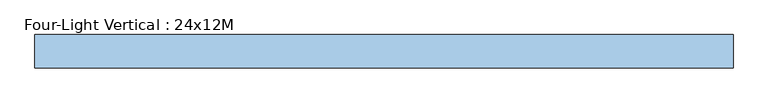
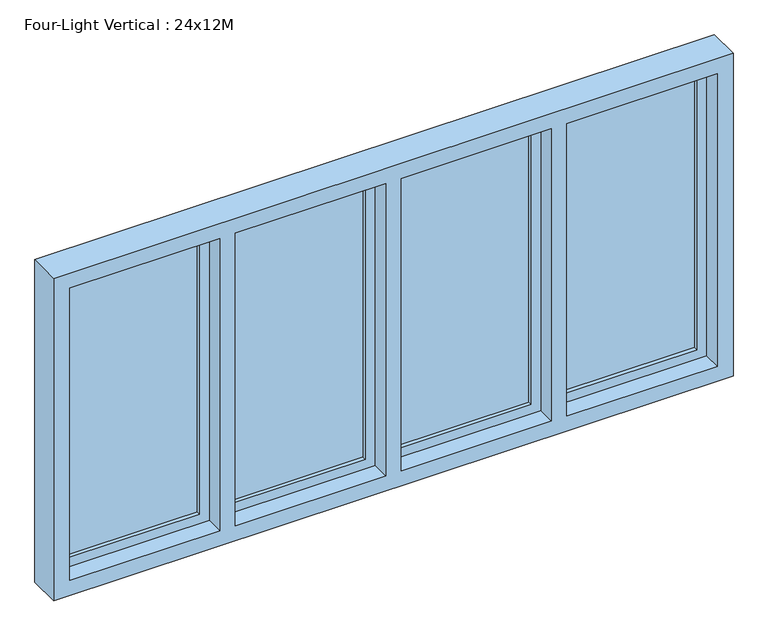
"""IFC4 building model written with IfcOpenShell, lengths in millimetres: window geometry, Four-Light Vertical : 24x12M."""

from ifc_helpers import new_model, si_unit, frame, origin, place, context, project, spatial, polyline, outline, extrude, faceted_brep, source, transform, mapped, element, save


def four_light_vertical_24x12m_47221696(model_context):
    return source(origin(), model_context, "Body", "SolidModel", [
        extrude(outline(polyline([(1970.0, -1224.0), (842.0, -1224.0), (842.0, -660.75), (1970.0, -660.75), (1970.0, -1224.0)]), holes=[polyline([(1920.0, -710.75), (892.0, -710.75), (892.0, -1174.0), (1920.0, -1174.0), (1920.0, -710.75)])]), frame((0.0, 134.0, 0.0), z_axis=(0.0, 1.0, 0.0), x_axis=(0.0, 0.0, 1.0)), (0.0, 0.0, 1.0), 50.0),
        extrude(outline(polyline([(1970.0, -635.75), (842.0, -635.75), (842.0, -72.5), (1970.0, -72.5), (1970.0, -635.75)]), holes=[polyline([(1920.0, -122.5), (892.0, -122.5), (892.0, -585.75), (1920.0, -585.75), (1920.0, -122.5)])]), frame((0.0, 134.0, 0.0), z_axis=(0.0, 1.0, 0.0), x_axis=(0.0, 0.0, 1.0)), (0.0, 0.0, 1.0), 50.0),
        extrude(outline(polyline([(1970.0, -47.5), (842.0, -47.5), (842.0, 515.75), (1970.0, 515.75), (1970.0, -47.5)]), holes=[polyline([(1920.0, 465.75), (892.0, 465.75), (892.0, 2.5), (1920.0, 2.5), (1920.0, 465.75)])]), frame((0.0, 134.0, 0.0), z_axis=(0.0, 1.0, 0.0), x_axis=(0.0, 0.0, 1.0)), (0.0, 0.0, 1.0), 50.0),
        extrude(outline(polyline([(1970.0, 540.75), (842.0, 540.75), (842.0, 1104.0), (1970.0, 1104.0), (1970.0, 540.75)]), holes=[polyline([(1920.0, 1054.0), (892.0, 1054.0), (892.0, 590.75), (1920.0, 590.75), (1920.0, 1054.0)])]), frame((0.0, 134.0, 0.0), z_axis=(0.0, 1.0, 0.0), x_axis=(0.0, 0.0, 1.0)), (0.0, 0.0, 1.0), 50.0),
        faceted_brep([(-1266.0, 184.0, 800.0), (1146.0, 184.0, 800.0), (1146.0, 69.0, 800.0), (-1266.0, 69.0, 800.0), (1146.0, 184.0, 2012.0), (1146.0, 69.0, 2012.0), (-1266.0, 184.0, 2012.0), (1104.0, 184.0, 842.0), (1104.0, 184.0, 1970.0), (540.75, 184.0, 1970.0), (540.75, 184.0, 842.0), (-1224.0, 184.0, 1970.0), (-1224.0, 184.0, 842.0), (-660.75, 184.0, 842.0), (-660.75, 184.0, 1970.0), (515.75, 184.0, 842.0), (515.75, 184.0, 1970.0), (-47.5, 184.0, 1970.0), (-47.5, 184.0, 842.0), (-72.5, 184.0, 1970.0), (-635.75, 184.0, 1970.0), (-635.75, 184.0, 842.0), (-72.5, 184.0, 842.0), (-1266.0, 69.0, 2012.0), (1089.0, 69.0, 1955.0), (1089.0, 69.0, 857.0), (555.75, 69.0, 857.0), (555.75, 69.0, 1955.0), (500.75, 69.0, 1955.0), (500.75, 69.0, 857.0), (-32.5, 69.0, 857.0), (-32.5, 69.0, 1955.0), (-87.5, 69.0, 857.0), (-620.75, 69.0, 857.0), (-620.75, 69.0, 1955.0), (-87.5, 69.0, 1955.0), (-1209.0, 69.0, 857.0), (-1209.0, 69.0, 1955.0), (-675.75, 69.0, 1955.0), (-675.75, 69.0, 857.0), (1089.0, 134.0, 857.0), (555.75, 134.0, 857.0), (-1209.0, 134.0, 857.0), (-675.75, 134.0, 857.0), (500.75, 134.0, 857.0), (-32.5, 134.0, 857.0), (-87.5, 134.0, 857.0), (-620.75, 134.0, 857.0), (1089.0, 134.0, 1955.0), (1104.0, 134.0, 1970.0), (1104.0, 134.0, 842.0), (540.75, 134.0, 842.0), (540.75, 134.0, 1970.0), (555.75, 134.0, 1955.0), (-1224.0, 134.0, 842.0), (-1224.0, 134.0, 1970.0), (-660.75, 134.0, 1970.0), (-660.75, 134.0, 842.0), (-1209.0, 134.0, 1955.0), (-675.75, 134.0, 1955.0), (515.75, 134.0, 1970.0), (515.75, 134.0, 842.0), (-47.5, 134.0, 842.0), (-47.5, 134.0, 1970.0), (500.75, 134.0, 1955.0), (-32.5, 134.0, 1955.0), (-72.5, 134.0, 1970.0), (-72.5, 134.0, 842.0), (-635.75, 134.0, 842.0), (-635.75, 134.0, 1970.0), (-87.5, 134.0, 1955.0), (-620.75, 134.0, 1955.0)], [[[0, 1, 2, 3]], [[2, 1, 4, 5]], [[4, 1, 0, 6], [7, 8, 9, 10], [11, 12, 13, 14], [15, 16, 17, 18], [19, 20, 21, 22]], [[2, 5, 23, 3], [24, 25, 26, 27], [28, 29, 30, 31], [32, 33, 34, 35], [36, 37, 38, 39]], [[25, 40, 41, 26]], [[42, 36, 39, 43]], [[29, 44, 45, 30]], [[32, 46, 47, 33]], [[40, 25, 24, 48]], [[49, 50, 51, 52], [40, 48, 53, 41]], [[54, 55, 56, 57], [58, 42, 43, 59]], [[60, 61, 62, 63], [44, 64, 65, 45]], [[66, 67, 68, 69], [46, 70, 71, 47]], [[68, 67, 22, 21]], [[50, 7, 10, 51]], [[12, 54, 57, 13]], [[61, 15, 18, 62]], [[7, 50, 49, 8]], [[23, 6, 0, 3]], [[58, 37, 36, 42]], [[11, 55, 54, 12]], [[10, 9, 52, 51]], [[27, 26, 41, 53]], [[29, 28, 64, 44]], [[16, 15, 61, 60]], [[18, 17, 63, 62]], [[31, 30, 45, 65]], [[32, 35, 70, 46]], [[19, 22, 67, 66]], [[21, 20, 69, 68]], [[34, 33, 47, 71]], [[39, 38, 59, 43]], [[14, 13, 57, 56]], [[23, 5, 4, 6]], [[48, 24, 27, 53]], [[37, 58, 59, 38]], [[64, 28, 31, 65]], [[70, 35, 34, 71]], [[8, 49, 52, 9]], [[16, 60, 63, 17]], [[19, 66, 69, 20]], [[56, 55, 11, 14]]]),
        extrude(outline(polyline([(2.5, 170.0), (465.75, 170.0), (465.75, 148.0), (2.5, 148.0), (2.5, 170.0)])), frame((0.0, 0.0, 892.0), z_axis=(0.0, 0.0, 1.0), x_axis=(1.0, 0.0, 0.0)), (0.0, 0.0, 1.0), 1028.0),
        extrude(outline(polyline([(-585.75, 170.0), (-122.5, 170.0), (-122.5, 148.0), (-585.75, 148.0), (-585.75, 170.0)])), frame((0.0, 0.0, 892.0), z_axis=(0.0, 0.0, 1.0), x_axis=(1.0, 0.0, 0.0)), (0.0, 0.0, 1.0), 1028.0),
        extrude(outline(polyline([(-1174.0, 170.0), (-710.75, 170.0), (-710.75, 148.0), (-1174.0, 148.0), (-1174.0, 170.0)])), frame((0.0, 0.0, 892.0), z_axis=(0.0, 0.0, 1.0), x_axis=(1.0, 0.0, 0.0)), (0.0, 0.0, 1.0), 1028.0),
        extrude(outline(polyline([(590.75, 170.0), (1054.0, 170.0), (1054.0, 148.0), (590.75, 148.0), (590.75, 170.0)])), frame((0.0, 0.0, 892.0), z_axis=(0.0, 0.0, 1.0), x_axis=(1.0, 0.0, 0.0)), (0.0, 0.0, 1.0), 1028.0),
    ])


if __name__ == "__main__":
    model = new_model("IFC4")
    model_context = context("Model", 3, world=origin())
    ifc_project = project(units=[si_unit("LENGTHUNIT", "METRE", prefix="MILLI")], contexts=[model_context])
    site = spatial("IfcSite", under=ifc_project)
    building = spatial("IfcBuilding", under=site)
    placement = place(None, origin())
    four_light_vertical_24x12m_shape = four_light_vertical_24x12m_47221696(model_context)
    element("IfcWindow", 1, ObjectType="Four-Light Vertical : 24x12M", at=placement, inside=building, context=model_context, shape_type="MappedRepresentation", body=[
        mapped(four_light_vertical_24x12m_shape, transform((0.0, 0.0, 0.0), x_axis=(1.0, 0.0, 0.0), y_axis=(0.0, 1.0, 0.0), z_axis=(0.0, 0.0, 1.0))),
    ])
    save(model, "model.ifc")

# Revit data of these elements
# Type "Four-Light Vertical : 24x12M"
#   Type Mark = "53"
#   Creator Organization [instance default] = "© Danish Educational Content"
#   Creator Name [instance default] = "© Erik Falck Jørgensen"
#   Creator Build [instance default] = "2017.0801.0"
#   Analytic Construction = "<None>"
#   length#6 = -36 mm
#   length#5 = -14 mm
#   length#3 = 29.5 mm
#   length#2 = 57 mm
#   length#1 = 0 mm
#   length#4 = 120 mm
#   Seal Width = 12 mm
#   Rough Width = 2412 mm
#   Rough Height = 1212 mm
#   Rebate Depth = 50 mm
#   Transom Width = 55 mm
#   Rabbet Width = 15 mm
#   Rabbet Depth = 50 mm
#   Height = 1188 mm
#   Glass Thickness = 22 mm
#   Frame Width = 50 mm
#   Frame Depth = 50 mm
#   Exterior Direction [instance default] = 0.00°
#   Case Depth = 115 mm
#   Case Width = 45 mm
#   Default Sill Height = 800 mm
#   Width = 2388 mm
#   Sealing = no
#   Hinging = yes
#   Wall Closure = 1
#   Above Cutplane [instance default] = no
#   Glass = none
#   Case/Transom = none
#   Frame/Mullion = none
#   Assembly Code = ""
# Element 1 (IfcWindow, "Four-Light Vertical : 24x12M")
#   Materials on its faces: "Default Frame/Mullion (Interior/Exterior)", "Glass"
# Materials
#   "Default Frame/Mullion (Interior/Exterior)": class "Generic", colour RGB 205 205 205, transparency 0, Description = "Udefineret karm/ramme materiale", Cost = 0
#   "Glass": class "Glass", colour RGB 180 200 255, transparency 0.75, Description = "Generisk glas", Cost = 0
